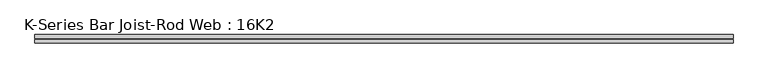
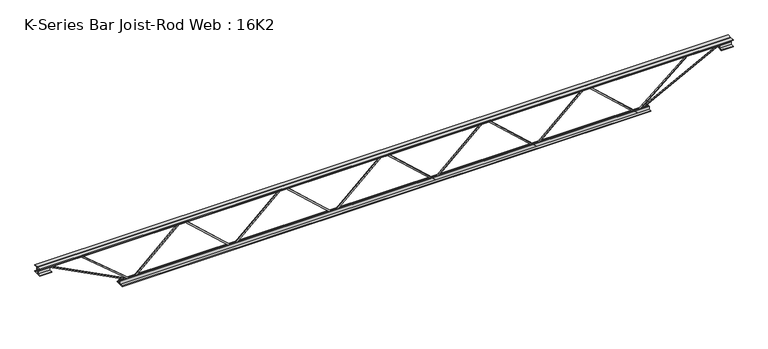
"""IFC4 building model written with IfcOpenShell, lengths in millimetres: beam geometry, K-Series Bar Joist-Rod Web : 16K2."""

from ifc_helpers import new_model, si_unit, frame, origin, place, context, project, spatial, polyline, outline, extrude, source, transform, mapped, element, save


def k_series_bar_joist_rod_web_16k2_80297fe6(model_context):
    return source(origin(), model_context, "Body", "SweptSolid", [
        extrude(outline(polyline([(-192.0875, 436.88), (-201.6125, 436.88), (-201.6125, 441.9042361), (192.0875, 872.4342361), (192.0875, 875.0857639), (-201.6125, 1305.6157639), (-201.6125, 1310.64), (-192.0875, 1310.64), (-192.0875, 1309.3142361), (201.6125, 878.7842361), (201.6125, 868.7357639), (-192.0875, 438.2057639), (-192.0875, 436.88)])), frame((0.0, -4.7625, 0.0), z_axis=(0.0, 1.0, 0.0), x_axis=(0.0, 0.0, 1.0)), (0.0, 0.0, 1.0), 9.525),
        extrude(outline(polyline([(-192.0875, -436.88), (-201.6125, -436.88), (-201.6125, -431.8557639), (192.0875, -1.3257639), (192.0875, 1.3257639), (-201.6125, 431.8557639), (-201.6125, 436.88), (-192.0875, 436.88), (-192.0875, 435.5542361), (201.6125, 5.0242361), (201.6125, -5.0242361), (-192.0875, -435.5542361), (-192.0875, -436.88)])), frame((0.0, -4.7625, 0.0), z_axis=(0.0, 1.0, 0.0), x_axis=(0.0, 0.0, 1.0)), (0.0, 0.0, 1.0), 9.525),
        extrude(outline(polyline([(-192.0875, -1310.64), (-201.6125, -1310.64), (-201.6125, -1305.6157639), (192.0875, -875.0857639), (192.0875, -872.4342361), (-201.6125, -441.9042361), (-201.6125, -436.88), (-192.0875, -436.88), (-192.0875, -438.2057639), (201.6125, -868.7357639), (201.6125, -878.7842361), (-192.0875, -1309.3142361), (-192.0875, -1310.64)])), frame((0.0, -4.7625, 0.0), z_axis=(0.0, 1.0, 0.0), x_axis=(0.0, 0.0, 1.0)), (0.0, 0.0, 1.0), 9.525),
        extrude(outline(polyline([(-192.0875, 1310.64), (-201.6125, 1310.64), (-201.6125, 1315.6642361), (192.0875, 1746.1942361), (192.0875, 1748.8457639), (-201.6125, 2179.3757639), (-201.6125, 2184.4), (-192.0875, 2184.4), (-192.0875, 2183.0742361), (201.6125, 1752.5442361), (201.6125, 1742.4957639), (-192.0875, 1311.9657639), (-192.0875, 1310.64)])), frame((0.0, -4.7625, 0.0), z_axis=(0.0, 1.0, 0.0), x_axis=(0.0, 0.0, 1.0)), (0.0, 0.0, 1.0), 9.525),
        extrude(outline(polyline([(-192.0875, -2184.4), (-201.6125, -2184.4), (-201.6125, -2179.3757639), (192.0875, -1748.8457639), (192.0875, -1746.1942361), (-201.6125, -1315.6642361), (-201.6125, -1310.64), (-192.0875, -1310.64), (-192.0875, -1311.9657639), (201.6125, -1742.4957639), (201.6125, -1752.5442361), (-192.0875, -2183.0742361), (-192.0875, -2184.4)])), frame((0.0, -4.7625, 0.0), z_axis=(0.0, 1.0, 0.0), x_axis=(0.0, 0.0, 1.0)), (0.0, 0.0, 1.0), 9.525),
        extrude(outline(polyline([(4.7625, 203.2), (36.5125, 203.2), (36.5125, 196.85), (11.1125, 196.85), (11.1125, 171.45), (4.7625, 171.45), (4.7625, 203.2)])), frame((-2997.2, 0.0, 0.0), z_axis=(1.0, 0.0, 0.0), x_axis=(0.0, 1.0, 0.0)), (0.0, 0.0, 1.0), 5994.4),
        extrude(outline(polyline([(-4.7625, 203.2), (-4.7625, 171.45), (-11.1125, 171.45), (-11.1125, 196.85), (-36.5125, 196.85), (-36.5125, 203.2), (-4.7625, 203.2)])), frame((-2997.2, 0.0, 0.0), z_axis=(1.0, 0.0, 0.0), x_axis=(0.0, 1.0, 0.0)), (0.0, 0.0, 1.0), 5994.4),
        extrude(outline(polyline([(-4.7625, 139.7), (-36.5125, 139.7), (-36.5125, 146.05), (-11.1125, 146.05), (-11.1125, 171.45), (-4.7625, 171.45), (-4.7625, 139.7)])), frame((-2997.2, 0.0, 0.0), z_axis=(1.0, 0.0, 0.0), x_axis=(0.0, 1.0, 0.0)), (0.0, 0.0, 1.0), 101.6),
        extrude(outline(polyline([(36.5125, 139.7), (4.7625, 139.7), (4.7625, 171.45), (11.1125, 171.45), (11.1125, 146.05), (36.5125, 146.05), (36.5125, 139.7)])), frame((-2997.2, 0.0, 0.0), z_axis=(1.0, 0.0, 0.0), x_axis=(0.0, 1.0, 0.0)), (0.0, 0.0, 1.0), 101.6),
        extrude(outline(polyline([(4.7625, 139.7), (4.7625, 171.45), (11.1125, 171.45), (11.1125, 146.05), (36.5125, 146.05), (36.5125, 139.7), (4.7625, 139.7)])), frame((2895.6, 0.0, 0.0), z_axis=(1.0, 0.0, 0.0), x_axis=(0.0, 1.0, 0.0)), (0.0, 0.0, 1.0), 101.6),
        extrude(outline(polyline([(-4.7625, 139.7), (-36.5125, 139.7), (-36.5125, 146.05), (-11.1125, 146.05), (-11.1125, 171.45), (-4.7625, 171.45), (-4.7625, 139.7)])), frame((2895.6, 0.0, 0.0), z_axis=(1.0, 0.0, 0.0), x_axis=(0.0, 1.0, 0.0)), (0.0, 0.0, 1.0), 101.6),
        extrude(outline(polyline([(4.7625, -203.2), (4.7625, -171.45), (11.1125, -171.45), (11.1125, -196.85), (36.5125, -196.85), (36.5125, -203.2), (4.7625, -203.2)])), frame((-2286.0, 0.0, 0.0), z_axis=(1.0, 0.0, 0.0), x_axis=(0.0, 1.0, 0.0)), (0.0, 0.0, 1.0), 4572.0),
        extrude(outline(polyline([(-4.7625, -203.2), (-36.5125, -203.2), (-36.5125, -196.85), (-11.1125, -196.85), (-11.1125, -171.45), (-4.7625, -171.45), (-4.7625, -203.2)])), frame((-2286.0, 0.0, 0.0), z_axis=(1.0, 0.0, 0.0), x_axis=(0.0, 1.0, 0.0)), (0.0, 0.0, 1.0), 4572.0),
        extrude(outline(polyline([(0.0, -9.525), (0.0, 0.0), (800.9059433, 0.0), (800.9059433, -9.525), (0.0, -9.525)])), frame((-2897.7900559, 4.7625, 167.2209266), z_axis=(0.4598542476611367, 0.0, 0.8879944092774514), x_axis=(0.8879944092774514, 0.0, -0.4598542476611367)), (0.0, 0.0, 1.0), 9.525),
        extrude(outline(polyline([(0.0, -9.525), (0.0, 0.0), (571.4096818, 0.0), (571.4096818, -9.525), (0.0, -9.525)])), frame((-2624.3496518, 4.7625, 167.8087579), z_axis=(0.6445463067243395, 0.0, 0.764565274183973), x_axis=(0.764565274183973, 0.0, -0.6445463067243395)), (0.0, 0.0, 1.0), 9.525),
        extrude(outline(polyline([(0.0, -9.525), (0.0, 0.0), (800.9059433, 0.0), (800.9059433, -9.525), (0.0, -9.525)])), frame((2897.7900559, -4.7625, 167.2209266), z_axis=(-0.4598542476611247, 0.0, 0.8879944092774577), x_axis=(-0.8879944092774577, 0.0, -0.4598542476611247)), (0.0, 0.0, 1.0), 9.525),
        extrude(outline(polyline([(0.0, -9.525), (0.0, 0.0), (571.4096818, 0.0), (571.4096818, -9.525), (0.0, -9.525)])), frame((2624.3496518, -4.7625, 167.8087579), z_axis=(-0.6445463067243351, 0.0, 0.7645652741839766), x_axis=(-0.7645652741839766, 0.0, -0.6445463067243351)), (0.0, 0.0, 1.0), 9.525),
    ])


if __name__ == "__main__":
    model = new_model("IFC4")
    model_context = context("Model", 3, world=origin())
    ifc_project = project(units=[si_unit("LENGTHUNIT", "METRE", prefix="MILLI")], contexts=[model_context])
    site = spatial("IfcSite", under=ifc_project)
    building = spatial("IfcBuilding", under=site)
    placement = place(None, origin())
    k_series_bar_joist_rod_web_16k2_shape = k_series_bar_joist_rod_web_16k2_80297fe6(model_context)
    element("IfcBeam", 1, ObjectType="K-Series Bar Joist-Rod Web : 16K2", at=placement, inside=building, context=model_context, shape_type="MappedRepresentation", body=[
        mapped(k_series_bar_joist_rod_web_16k2_shape, transform((0.0, 0.0, 0.0), x_axis=(1.0, 0.0, 0.0), y_axis=(0.0, 1.0, 0.0), z_axis=(0.0, 0.0, 1.0))),
    ])
    save(model, "model.ifc")

# Revit data of these elements
# Type "K-Series Bar Joist-Rod Web : 16K2"
#   Assembly Code = "B1010350"
#   Wt = 5.5
#   Web Thickness = 0' - 0 3/8"
#   Start Offset [instance default] = 0' - 0"
#   Start Extension [instance default] = 0' - 0"
#   Seat Length = 0' - 4"
#   Seat Depth = 0' - 2 1/2"
#   PanelArrayLength [instance default] = 18' - 8"
#   Panel [instance default] = 2' - 8"
#   End Offset [instance default] = 0' - 0"
#   End Extension [instance default] = 0' - 0"
#   End Panel = 2' - 8"
#   Cord Leg = 0' - 1 1/4"
#   Chord Thickness = 0' - 0 1/4"
#   Length [instance default] = 24' - 0"
#   Depth = 1' - 4"
#   PanelArrayNum [instance default] = 7
#   Structural Material = none
# Element 1 (IfcBeam, "K-Series Bar Joist-Rod Web : 16K2")
#   PanelArrayLength = 14' - 4"
#   Panel = 2' - 10.4"
#   PanelArrayNum = 5
